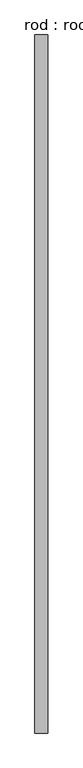
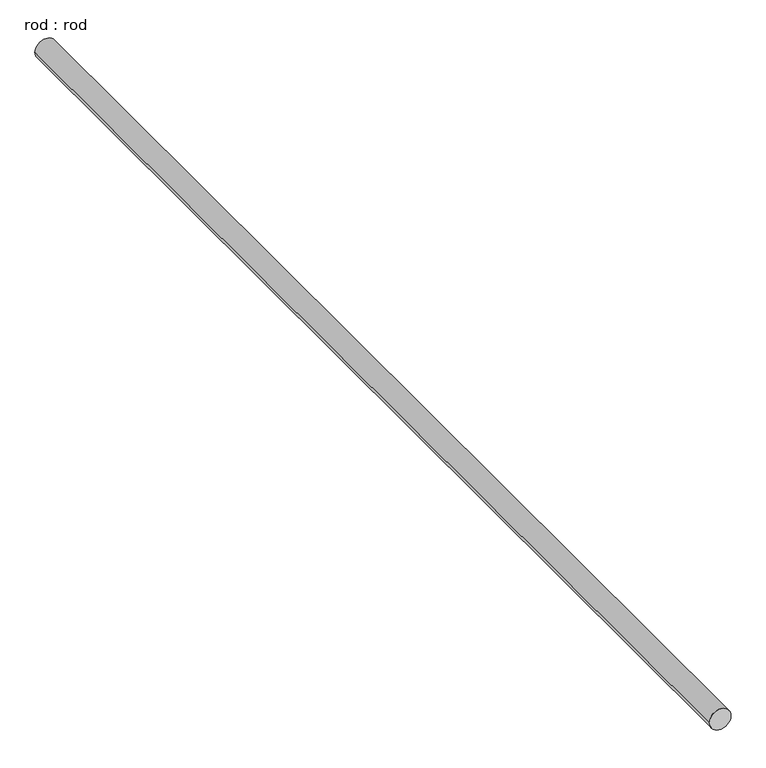
"""IFC4 building model written with IfcOpenShell, lengths in millimetres: proxy geometry, rod : rod."""

from ifc_helpers import new_model, si_unit, point, frame, frame_2d, origin, place, context, project, spatial, circle_curve, trimmed, segment, composite_curve, outline, extrude, source, transform, mapped, element, save


def rod_rod_363700de(model_context):
    return source(origin(), model_context, "Body", "SweptSolid", [
        extrude(outline(composite_curve([segment(trimmed(circle_curve(frame_2d((0.0108462, 0.0)), 200.0), [point((0.0108462, 200.0))], [point((0.0108462, -200.0))], False, "CARTESIAN"), True, "CONTINUOUS"), segment(trimmed(circle_curve(frame_2d((0.0108462, 0.0)), 200.0), [point((0.0108462, -200.0))], [point((0.0108462, 200.0))], False, "CARTESIAN"), True, "CONTINUOUS")], self_intersect=False)), frame((0.0, -6672.1498338, 0.0), z_axis=(0.0, 1.0, 0.0), x_axis=(0.0, 0.0, 1.0)), (0.0, 0.0, 1.0), 21529.7568983),
    ])


if __name__ == "__main__":
    model = new_model("IFC4")
    model_context = context("Model", 3, world=origin())
    ifc_project = project(units=[si_unit("LENGTHUNIT", "METRE", prefix="MILLI")], contexts=[model_context])
    site = spatial("IfcSite", under=ifc_project)
    building = spatial("IfcBuilding", under=site)
    placement = place(None, origin())
    rod_rod_shape = rod_rod_363700de(model_context)
    element("IfcBuildingElementProxy", 1, Name="rod : rod", ObjectType="rod : rod", at=placement, inside=building, context=model_context, shape_type="MappedRepresentation", body=[
        mapped(rod_rod_shape, transform((0.0, 0.0, 0.0), x_axis=(1.0, 0.0, 0.0), y_axis=(0.0, 1.0, 0.0), z_axis=(0.0, 0.0, 1.0))),
    ])
    save(model, "model.ifc")

# Revit data of these elements
# Type "rod : rod"
#   Default Elevation = 0
